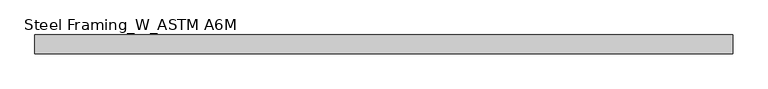
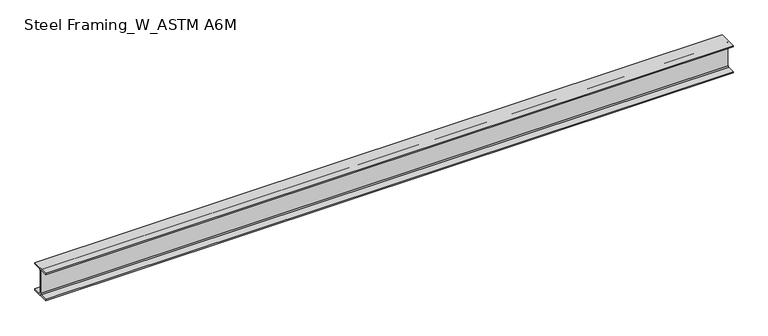
"""IFC4 building model written with IfcOpenShell, lengths in millimetres: beam geometry, Steel Framing_W_ASTM A6M : H_SB_AR_S02_W200x31.3_RB4."""

from ifc_helpers import new_model, si_unit, point, frame, frame_2d, origin, place, context, project, spatial, polyline, circle_curve, trimmed, segment, composite_curve, outline, extrude, source, transform, mapped, element, save


def steel_framing_w_astm_a6m_99937224(model_context):
    return source(origin(), model_context, "Body", "SweptSolid", [
        extrude(outline(composite_curve([segment(polyline([(67.0, -94.8), (67.0, -105.0), (-67.0, -105.0), (-67.0, -94.8), (-10.775, -94.8)]), True, "CONTINUOUS"), segment(trimmed(circle_curve(frame_2d((-10.775, -87.2)), 7.6), [point((-10.775, -94.8))], [point((-3.175, -87.2))], True, "CARTESIAN"), True, "CONTINUOUS"), segment(polyline([(-3.175, -87.2), (-3.175, 87.2)]), True, "CONTINUOUS"), segment(trimmed(circle_curve(frame_2d((-10.775, 87.2)), 7.6), [point((-3.175, 87.2))], [point((-10.775, 94.8))], True, "CARTESIAN"), True, "CONTINUOUS"), segment(polyline([(-10.775, 94.8), (-67.0, 94.8), (-67.0, 105.0), (67.0, 105.0), (67.0, 94.8), (10.775, 94.8)]), True, "CONTINUOUS"), segment(trimmed(circle_curve(frame_2d((10.775, 87.2)), 7.6), [point((10.775, 94.8))], [point((3.175, 87.2))], True, "CARTESIAN"), True, "CONTINUOUS"), segment(polyline([(3.175, 87.2), (3.175, -87.2)]), True, "CONTINUOUS"), segment(trimmed(circle_curve(frame_2d((10.775, -87.2)), 7.6), [point((3.175, -87.2))], [point((10.775, -94.8))], True, "CARTESIAN"), True, "CONTINUOUS"), segment(polyline([(10.775, -94.8), (67.0, -94.8)]), True, "CONTINUOUS")], self_intersect=False)), frame((-2487.2, 0.0, 0.0), z_axis=(1.0, 0.0, 0.0), x_axis=(0.0, 1.0, 0.0)), (0.0, 0.0, 1.0), 4974.4),
    ])


if __name__ == "__main__":
    model = new_model("IFC4")
    model_context = context("Model", 3, world=origin())
    ifc_project = project(units=[si_unit("LENGTHUNIT", "METRE", prefix="MILLI")], contexts=[model_context])
    site = spatial("IfcSite", under=ifc_project)
    building = spatial("IfcBuilding", under=site)
    placement = place(None, origin())
    steel_framing_w_astm_a6m_shape = steel_framing_w_astm_a6m_99937224(model_context)
    element("IfcBeam", 1, ObjectType="Steel Framing_W_ASTM A6M : H_SB_AR_S02_W200x31.3_RB4", at=placement, inside=building, context=model_context, shape_type="MappedRepresentation", body=[
        mapped(steel_framing_w_astm_a6m_shape, transform((0.0, 0.0, 0.0), x_axis=(1.0, 0.0, 0.0), y_axis=(0.0, 1.0, 0.0), z_axis=(0.0, 0.0, 1.0))),
    ])
    save(model, "model.ifc")

# Revit data of these elements
# Type "Steel Framing_W_ASTM A6M : H_SB_AR_S02_W200x31.3_RB4"
#   Type Mark = "RB4"
#   Section Name Key = "W8x21"
#   Width = 13.4 cm
#   Web Thickness = 0.635 cm
#   Web Fillet = 0.76 cm
#   Warping Constant = 40800.0 cm⁶
#   Torsional Moment of Inertia = 11.70 cm⁴
#   Section Area = 39.7 cm²
#   Plastic Modulus weak axis = 93.2 cm³
#   Plastic Modulus strong axis = 334.0 cm³
#   Perimeter = 0.93 m²/m
#   Nominal Weight = 31.30 kgf/m
#   Moment of Inertia weak axis = 407.00 cm⁴
#   Moment of Inertia strong axis = 3130.00 cm⁴
#   Height = 21.0 cm
#   Flange Thickness = 1.02 cm
#   Elastic Modulus weak axis = 60.8 cm³
#   Elastic Modulus strong axis = 298.0 cm³
#   Centroid Vertical = 10.5 cm
#   Centroid Horizontal = 6.7 cm
#   Length [instance default] = 1500 mm
#   Structural Material [instance default] = Steel, 45-345
#   Bolt Spacing = 0
#   Assembly Code = ""
# Element 1 (IfcBeam, "Steel Framing_W_ASTM A6M : H_SB_AR_S02_W200x31.3_RB4")
#   Materials on its faces: "Steel, 45-345"
# Materials
#   "Steel, 45-345": class "Metal", colour RGB 189 187 185, transparency 0, Description = "Steel 345 MPa", Cost = 0
